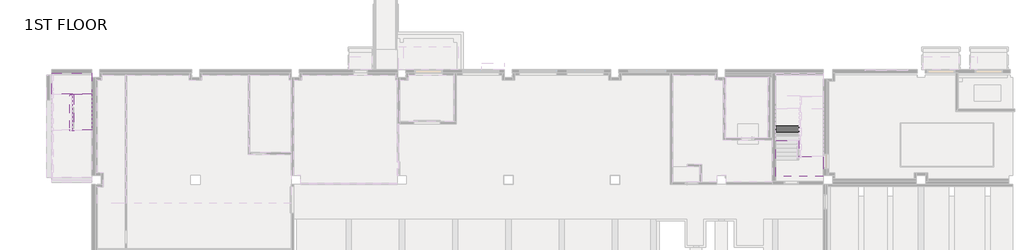
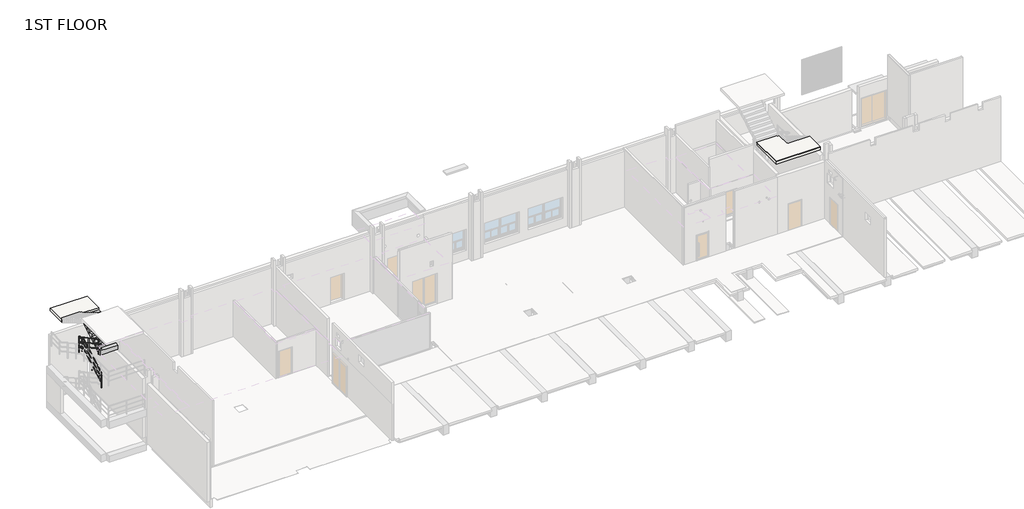
# One storey, part 13 of 15: 3 slabs, 2 stair flights, 1 railing.
"""IFC4 building model written with IfcOpenShell, lengths in millimetres."""

from ifc_helpers import new_model, si_unit, point, frame, frame_2d, origin, place, context, project, spatial, polyline, circle_curve, ellipse_curve, trimmed, segment, composite_curve, outline, extrude, faceted_brep, element, save
from ifc_brep_helpers import plane_surface, cylinder_surface, advanced_brep

model = new_model("IFC4")

# Units and contexts
model_context = context("Model", 3, world=origin())
ifc_project = project(units=[si_unit("LENGTHUNIT", "METRE", prefix="MILLI")], contexts=[model_context])

# Site, building, storey
site = spatial("IfcSite", under=ifc_project)
building = spatial("IfcBuilding", under=site)
storey = spatial("IfcBuildingStorey", under=building, Name="1ST FLOOR", Elevation=4800.0)

# Railing
placement = place(None, origin())
element("IfcRailing", 1, ObjectType="H_RL_AR_S10_Steel Handrail_H1200_STAIR", at=placement, inside=storey, context=model_context, shape_type="SolidModel", body=[
    advanced_brep(
    [(-1656.0, -4300.0, 8823.1475961), (-1694.0, -4300.0, 8823.1475961), (-1656.0, -1695.134128, 10251.0), (-1694.0, -1695.134128, 10251.0), (-1656.0, -1581.0, 10251.0), (-1694.0, -1619.0, 10251.0), (-1868.0, -1581.0, 10251.0), (-1868.0, -1619.0, 10251.0), (-1906.0, -1680.865872, 10402.2888889), (-1944.0, -1680.865872, 10402.2888889), (-1944.0, -4104.865872, 11731.0), (-1906.0, -4104.865872, 11731.0), (-1944.0, -4319.0, 11731.0), (-1906.0, -4281.0, 11731.0), (-1675.0, -4319.0, 11731.0), (-1675.0, -4281.0, 11731.0), (-1868.0, -1581.0, 10402.2888889), (-1868.0, -1619.0, 10402.2888889), (-1944.0, -1581.0, 10402.2888889), (-1906.0, -1619.0, 10402.2888889)],
    [
        (0, 1, ellipse_curve(frame((-1675.0, -4300.0, 8823.1475961), z_axis=(0.0, -1.0, 0.0), x_axis=(0.0, 0.0, -1.0)), 21.6672187, 19.0)),
        (1, 0, ellipse_curve(frame((-1675.0, -4300.0, 8823.1475961), z_axis=(0.0, -1.0, 0.0), x_axis=(0.0, 0.0, -1.0)), 21.6672187, 19.0)),
        (0, 2),
        (2, 3, ellipse_curve(frame((-1675.0, -1695.134128, 10251.0), z_axis=(0.0, -0.9687364795192938, -0.24809198545814556), x_axis=(0.0, 0.24809198545814448, -0.9687364795192941)), 19.613177, 19.0)),
        (3, 1),
        (3, 2, ellipse_curve(frame((-1675.0, -1695.134128, 10251.0), z_axis=(0.0, -0.9687364795192938, -0.24809198545814556), x_axis=(0.0, 0.24809198545814448, -0.9687364795192941)), 19.613177, 19.0)),
        (2, 4),
        (4, 5, ellipse_curve(frame((-1675.0, -1600.0, 10251.0), z_axis=(0.7071067811865467, -0.7071067811865485, 0.0), x_axis=(-0.7071067811865485, -0.7071067811865465, 0.0)), 26.8700577, 19.0)),
        (5, 3),
        (5, 4, ellipse_curve(frame((-1675.0, -1600.0, 10251.0), z_axis=(0.7071067811865467, -0.7071067811865485, 0.0), x_axis=(-0.7071067811865485, -0.7071067811865465, 0.0)), 26.8700577, 19.0)),
        (4, 6),
        (6, 7, ellipse_curve(frame((-1868.0, -1600.0, 10251.0), z_axis=(0.7071067811865475, 0.0, -0.7071067811865475), x_axis=(0.7071067811865477, 0.0, 0.7071067811865474)), 26.8700577, 19.0)),
        (7, 5),
        (7, 6, ellipse_curve(frame((-1868.0, -1600.0, 10251.0), z_axis=(0.7071067811865475, 0.0, -0.7071067811865475), x_axis=(0.7071067811865477, 0.0, 0.7071067811865474)), 26.8700577, 19.0)),
        (8, 9, ellipse_curve(frame((-1925.0, -1680.865872, 10402.2888889), z_axis=(0.0, -0.9687364795192939, 0.24809198545814537), x_axis=(0.0, -0.24809198545814468, -0.9687364795192942)), 19.613177, 19.0)),
        (9, 10),
        (10, 11, ellipse_curve(frame((-1925.0, -4104.865872, 11731.0), z_axis=(0.0, 0.9687364795192939, -0.24809198545814534), x_axis=(0.0, -0.24809198545814465, -0.9687364795192941)), 19.613177, 19.0)),
        (11, 8),
        (9, 8, ellipse_curve(frame((-1925.0, -1680.865872, 10402.2888889), z_axis=(0.0, -0.9687364795192939, 0.24809198545814537), x_axis=(0.0, -0.24809198545814468, -0.9687364795192942)), 19.613177, 19.0)),
        (11, 10, ellipse_curve(frame((-1925.0, -4104.865872, 11731.0), z_axis=(0.0, 0.9687364795192939, -0.24809198545814534), x_axis=(0.0, -0.24809198545814465, -0.9687364795192941)), 19.613177, 19.0)),
        (10, 12),
        (12, 13, ellipse_curve(frame((-1925.0, -4300.0, 11731.0), z_axis=(-0.7071067811864243, 0.7071067811866708, 0.0), x_axis=(0.7071067811866707, 0.7071067811864242, 0.0)), 26.8700577, 19.0)),
        (13, 11),
        (13, 12, ellipse_curve(frame((-1925.0, -4300.0, 11731.0), z_axis=(-0.7071067811864243, 0.7071067811866708, 0.0), x_axis=(0.7071067811866707, 0.7071067811864242, 0.0)), 26.8700577, 19.0)),
        (14, 15, circle_curve(frame((-1675.0, -4300.0, 11731.0), z_axis=(1.0, 0.0, 0.0), x_axis=(0.0, 1.0, 0.0)), 19.0)),
        (15, 14, circle_curve(frame((-1675.0, -4300.0, 11731.0), z_axis=(1.0, 0.0, 0.0), x_axis=(0.0, 1.0, 0.0)), 19.0)),
        (12, 14),
        (15, 13),
        (6, 16),
        (16, 17, ellipse_curve(frame((-1868.0, -1600.0, 10402.2888889), z_axis=(0.7071067811865475, 0.0, -0.7071067811865475), x_axis=(-0.7071067811865474, 0.0, -0.7071067811865476)), 26.8700577, 19.0)),
        (17, 7),
        (17, 16, ellipse_curve(frame((-1868.0, -1600.0, 10402.2888889), z_axis=(0.7071067811865475, 0.0, -0.7071067811865475), x_axis=(-0.7071067811865474, 0.0, -0.7071067811865476)), 26.8700577, 19.0)),
        (16, 18),
        (18, 19, ellipse_curve(frame((-1925.0, -1600.0, 10402.2888889), z_axis=(0.70710678118664, 0.707106781186455, 0.0), x_axis=(0.707106781186455, -0.70710678118664, 0.0)), 26.8700577, 19.0)),
        (19, 17),
        (19, 18, ellipse_curve(frame((-1925.0, -1600.0, 10402.2888889), z_axis=(0.70710678118664, 0.707106781186455, 0.0), x_axis=(0.707106781186455, -0.70710678118664, 0.0)), 26.8700577, 19.0)),
        (18, 9),
        (8, 19),
    ],
    [
        plane_surface(frame((-1675.0, -4300.0, 8844.8148148), z_axis=(0.0, -1.0, 0.0), x_axis=(0.0, 0.0, 1.0))),
        cylinder_surface(frame((-1675.0, -4290.8672412, 8828.1537009), z_axis=(0.0, -0.8769007335028707, -0.48067151317935164), x_axis=(-1.0, 0.0, 0.0)), 19.0),
        cylinder_surface(frame((-1675.0, -1700.0, 10251.0), z_axis=(0.0, -1.0, 0.0), x_axis=(-1.0, 0.0, 0.0)), 19.0),
        cylinder_surface(frame((-1675.0, -1600.0, 10251.0), z_axis=(1.0, 0.0, 0.0), x_axis=(0.0, -1.0, 0.0)), 19.0),
        cylinder_surface(frame((-1925.0, -1685.1327588, 10404.627775), z_axis=(0.0, 0.8769007335028708, -0.48067151317935125), x_axis=(1.0, 0.0, 0.0)), 19.0),
        cylinder_surface(frame((-1925.0, -4100.0, 11731.0), z_axis=(0.0, 1.0, 0.0), x_axis=(1.0, 0.0, 0.0)), 19.0),
        plane_surface(frame((-1675.0, -4300.0, 11750.0), z_axis=(1.0, 0.0, 0.0), x_axis=(0.0, 1.0, 0.0))),
        cylinder_surface(frame((-1925.0, -4300.0, 11731.0), z_axis=(-1.0, 0.0, 0.0), x_axis=(0.0, 1.0, 0.0)), 19.0),
        cylinder_surface(frame((-1868.0, -1600.0, 10270.0), z_axis=(0.0, 0.0, -1.0), x_axis=(0.0, -1.0, 0.0)), 19.0),
        cylinder_surface(frame((-1849.0, -1600.0, 10402.2888889), z_axis=(1.0, 0.0, 0.0), x_axis=(0.0, -1.0, 0.0)), 19.0),
        cylinder_surface(frame((-1925.0, -1600.0, 10402.2888889), z_axis=(0.0, 1.0, 0.0), x_axis=(1.0, 0.0, 0.0)), 19.0),
    ],
    [
        (0, [[1, 2]]),
        (1, [[-1, 3, 4, 5]]),
        (1, [[-2, -5, 6, -3]]),
        (2, [[-4, 7, 8, 9]]),
        (2, [[-6, -9, 10, -7]]),
        (3, [[-8, 11, 12, 13]]),
        (3, [[-10, -13, 14, -11]]),
        (4, [[15, 16, 17, 18]]),
        (4, [[19, -18, 20, -16]]),
        (5, [[-17, 21, 22, 23]]),
        (5, [[-20, -23, 24, -21]]),
        (6, [[25, 26]]),
        (7, [[-22, 27, -26, 28]]),
        (7, [[-24, -28, -25, -27]]),
        (8, [[-12, 29, 30, 31]]),
        (8, [[-14, -31, 32, -29]]),
        (9, [[-30, 33, 34, 35]]),
        (9, [[-32, -35, 36, -33]]),
        (10, [[-34, 37, -15, 38]]),
        (10, [[-36, -38, -19, -37]]),
    ],
),
    advanced_brep(
    [(-1675.0, -4319.0, 10931.0), (-1675.0, -4281.0, 10931.0), (-1944.0, -4319.0, 10931.0), (-1906.0, -4281.0, 10931.0)],
    [
        (0, 1, circle_curve(frame((-1675.0, -4300.0, 10931.0), z_axis=(1.0, 0.0, 0.0), x_axis=(0.0, 1.0, 0.0)), 19.0)),
        (1, 0, circle_curve(frame((-1675.0, -4300.0, 10931.0), z_axis=(1.0, 0.0, 0.0), x_axis=(0.0, 1.0, 0.0)), 19.0)),
        (2, 3, ellipse_curve(frame((-1925.0, -4300.0, 10931.0), z_axis=(-0.7071067811865471, 0.7071067811865479, 0.0), x_axis=(0.7071067811865479, 0.7071067811865471, 0.0)), 26.8700577, 19.0)),
        (3, 2, ellipse_curve(frame((-1925.0, -4300.0, 10931.0), z_axis=(-0.7071067811865471, 0.7071067811865479, 0.0), x_axis=(0.7071067811865479, 0.7071067811865471, 0.0)), 26.8700577, 19.0)),
        (0, 2),
        (3, 1),
    ],
    [
        plane_surface(frame((-1675.0, -4300.0, 10950.0), z_axis=(1.0, 0.0, 0.0), x_axis=(0.0, -1.0, 0.0))),
        plane_surface(frame((-1925.0, -4300.0, 10950.0), z_axis=(-0.7071067811865471, 0.7071067811865479, 0.0), x_axis=(0.7071067811865479, 0.7071067811865471, 0.0))),
        cylinder_surface(frame((-1675.0, -4300.0, 10931.0), z_axis=(1.0, 0.0, 0.0), x_axis=(0.0, 1.0, 0.0)), 19.0),
    ],
    [
        (0, [[1, 2]]),
        (1, [[3, 4]]),
        (2, [[-1, 5, -4, 6]]),
        (2, [[-2, -6, -3, -5]]),
    ],
),
    advanced_brep(
    [(-1944.0, -4319.0, 10931.0), (-1906.0, -4281.0, 10931.0), (-1944.0, -4104.865872, 10931.0), (-1906.0, -4104.865872, 10931.0), (-1944.0, -1592.4716448, 9553.8357569), (-1906.0, -1625.7938727, 9572.1012744)],
    [
        (0, 1, ellipse_curve(frame((-1925.0, -4300.0, 10931.0), z_axis=(0.7071067811865471, -0.7071067811865479, 0.0), x_axis=(-0.7071067811865478, -0.7071067811865472, 0.0)), 26.8700577, 19.0)),
        (1, 0, ellipse_curve(frame((-1925.0, -4300.0, 10931.0), z_axis=(0.7071067811865471, -0.7071067811865479, 0.0), x_axis=(-0.7071067811865478, -0.7071067811865472, 0.0)), 26.8700577, 19.0)),
        (0, 2),
        (2, 3, ellipse_curve(frame((-1925.0, -4104.865872, 10931.0), z_axis=(0.0, -0.9687364795192939, 0.24809198545814531), x_axis=(0.0, -0.24809198545814604, -0.9687364795192938)), 19.613177, 19.0)),
        (3, 1),
        (3, 2, ellipse_curve(frame((-1925.0, -4104.865872, 10931.0), z_axis=(0.0, -0.9687364795192939, 0.24809198545814531), x_axis=(0.0, -0.24809198545814604, -0.9687364795192938)), 19.613177, 19.0)),
        (4, 5, ellipse_curve(frame((-1925.0, -1609.1327588, 9562.9685157), z_axis=(0.7071067811865346, 0.6200624550873559, -0.33988608649231156), x_axis=(0.7071067811865606, -0.6200624550873189, 0.33988608649232477)), 26.8700577, 19.0)),
        (5, 4, ellipse_curve(frame((-1925.0, -1609.1327588, 9562.9685157), z_axis=(0.7071067811865346, 0.6200624550873559, -0.33988608649231156), x_axis=(0.7071067811865606, -0.6200624550873189, 0.33988608649232477)), 26.8700577, 19.0)),
        (2, 4),
        (5, 3),
    ],
    [
        plane_surface(frame((-1925.0, -4300.0, 10950.0), z_axis=(0.7071067811865471, -0.7071067811865479, 0.0), x_axis=(0.7071067811865479, 0.7071067811865471, 0.0))),
        cylinder_surface(frame((-1925.0, -4300.0, 10931.0), z_axis=(0.0, -1.0, 0.0), x_axis=(1.0, 0.0, 0.0)), 19.0),
        plane_surface(frame((-1925.0, -1600.0, 9579.6296296), z_axis=(0.7071067811865346, 0.6200624550873559, -0.33988608649231156), x_axis=(0.7071067811865605, -0.6200624550873332, 0.33988608649229907))),
        cylinder_surface(frame((-1925.0, -4109.1327588, 10933.3388861), z_axis=(0.0, -0.8769007335028708, 0.4806715131793512), x_axis=(1.0, 0.0, 0.0)), 19.0),
    ],
    [
        (0, [[1, 2]]),
        (1, [[-1, 3, 4, 5]]),
        (1, [[-2, -5, 6, -3]]),
        (2, [[7, 8]]),
        (3, [[-4, 9, -8, 10]]),
        (3, [[-6, -10, -7, -9]]),
    ],
),
    advanced_brep(
    [(-1950.7938727, -1581.0, 9451.0), (-1917.4716448, -1619.0, 9451.0), (-1656.0, -1581.0, 9451.0), (-1694.0, -1619.0, 9451.0)],
    [
        (0, 1, ellipse_curve(frame((-1934.1327587, -1600.0, 9451.0), z_axis=(-0.7071067811865346, -0.6200624550873559, 0.33988608649231156), x_axis=(-0.7071067811865603, 0.6200624550873332, -0.33988608649229907)), 26.8700577, 19.0)),
        (1, 0, ellipse_curve(frame((-1934.1327587, -1600.0, 9451.0), z_axis=(-0.7071067811865346, -0.6200624550873559, 0.33988608649231156), x_axis=(-0.7071067811865603, 0.6200624550873332, -0.33988608649229907)), 26.8700577, 19.0)),
        (2, 3, ellipse_curve(frame((-1675.0, -1600.0, 9451.0), z_axis=(0.7071067811865619, -0.7071067811865331, 0.0), x_axis=(-0.7071067811865331, -0.7071067811865619, 0.0)), 26.8700577, 19.0)),
        (3, 2, ellipse_curve(frame((-1675.0, -1600.0, 9451.0), z_axis=(0.7071067811865619, -0.7071067811865331, 0.0), x_axis=(-0.7071067811865331, -0.7071067811865619, 0.0)), 26.8700577, 19.0)),
        (0, 2),
        (3, 1),
    ],
    [
        plane_surface(frame((-1925.0, -1600.0, 9470.0), z_axis=(-0.7071067811865346, -0.6200624550873559, 0.33988608649231156), x_axis=(0.7071067811865605, -0.6200624550873332, 0.33988608649229907))),
        plane_surface(frame((-1675.0, -1600.0, 9470.0), z_axis=(0.7071067811865619, -0.7071067811865331, 0.0), x_axis=(0.7071067811865331, 0.7071067811865619, 0.0))),
        cylinder_surface(frame((-1925.0, -1600.0, 9451.0), z_axis=(-1.0, 0.0, 0.0), x_axis=(0.0, -1.0, 0.0)), 19.0),
    ],
    [
        (0, [[1, 2]]),
        (1, [[3, 4]]),
        (2, [[-1, 5, -4, 6]]),
        (2, [[-2, -6, -3, -5]]),
    ],
),
    advanced_brep(
    [(-1656.0, -1581.0, 9451.0), (-1694.0, -1619.0, 9451.0), (-1656.0, -1695.134128, 9451.0), (-1694.0, -1695.134128, 9451.0), (-1656.0, -4300.0, 8023.1475961), (-1694.0, -4300.0, 8023.1475961)],
    [
        (0, 1, ellipse_curve(frame((-1675.0, -1600.0, 9451.0), z_axis=(-0.7071067811865619, 0.7071067811865331, 0.0), x_axis=(0.707106781186533, 0.7071067811865619, 0.0)), 26.8700577, 19.0)),
        (1, 0, ellipse_curve(frame((-1675.0, -1600.0, 9451.0), z_axis=(-0.7071067811865619, 0.7071067811865331, 0.0), x_axis=(0.707106781186533, 0.7071067811865619, 0.0)), 26.8700577, 19.0)),
        (0, 2),
        (2, 3, ellipse_curve(frame((-1675.0, -1695.134128, 9451.0), z_axis=(0.0, 0.9687364795192939, 0.24809198545814562), x_axis=(0.0, 0.24809198545814576, -0.9687364795192939)), 19.613177, 19.0)),
        (3, 1),
        (3, 2, ellipse_curve(frame((-1675.0, -1695.134128, 9451.0), z_axis=(0.0, 0.9687364795192939, 0.24809198545814562), x_axis=(0.0, 0.24809198545814576, -0.9687364795192939)), 19.613177, 19.0)),
        (4, 5, ellipse_curve(frame((-1675.0, -4300.0, 8023.1475961), z_axis=(0.0, -1.0, 0.0), x_axis=(0.0, 0.0, 0.9999999999999999)), 21.6672187, 19.0)),
        (5, 4, ellipse_curve(frame((-1675.0, -4300.0, 8023.1475961), z_axis=(0.0, -1.0, 0.0), x_axis=(0.0, 0.0, 0.9999999999999999)), 21.6672187, 19.0)),
        (2, 4),
        (5, 3),
    ],
    [
        plane_surface(frame((-1675.0, -1600.0, 9470.0), z_axis=(-0.7071067811865619, 0.7071067811865331, 0.0), x_axis=(0.7071067811865331, 0.7071067811865619, 0.0))),
        cylinder_surface(frame((-1675.0, -1600.0, 9451.0), z_axis=(0.0, 1.0, 0.0), x_axis=(-1.0, 0.0, 0.0)), 19.0),
        plane_surface(frame((-1675.0, -4300.0, 8044.8148148), z_axis=(0.0, -1.0, 0.0), x_axis=(0.0, 0.0, -1.0))),
        cylinder_surface(frame((-1675.0, -1690.8672412, 9453.3388861), z_axis=(0.0, 0.8769007335028706, 0.4806715131793517), x_axis=(-1.0, 0.0, 0.0)), 19.0),
    ],
    [
        (0, [[1, 2]]),
        (1, [[-1, 3, 4, 5]]),
        (1, [[-2, -5, 6, -3]]),
        (2, [[7, 8]]),
        (3, [[-4, 9, -8, 10]]),
        (3, [[-6, -10, -7, -9]]),
    ],
),
    advanced_brep(
    [(-1675.0, -4319.0, 11331.0), (-1675.0, -4281.0, 11331.0), (-1944.0, -4319.0, 11331.0), (-1906.0, -4281.0, 11331.0)],
    [
        (0, 1, circle_curve(frame((-1675.0, -4300.0, 11331.0), z_axis=(1.0, 0.0, 0.0), x_axis=(0.0, 1.0, 0.0)), 19.0)),
        (1, 0, circle_curve(frame((-1675.0, -4300.0, 11331.0), z_axis=(1.0, 0.0, 0.0), x_axis=(0.0, 1.0, 0.0)), 19.0)),
        (2, 3, ellipse_curve(frame((-1925.0, -4300.0, 11331.0), z_axis=(-0.7071067811865471, 0.7071067811865479, 0.0), x_axis=(0.7071067811865479, 0.7071067811865471, 0.0)), 26.8700577, 19.0)),
        (3, 2, ellipse_curve(frame((-1925.0, -4300.0, 11331.0), z_axis=(-0.7071067811865471, 0.7071067811865479, 0.0), x_axis=(0.7071067811865479, 0.7071067811865471, 0.0)), 26.8700577, 19.0)),
        (0, 2),
        (3, 1),
    ],
    [
        plane_surface(frame((-1675.0, -4300.0, 11350.0), z_axis=(1.0, 0.0, 0.0), x_axis=(0.0, -1.0, 0.0))),
        plane_surface(frame((-1925.0, -4300.0, 11350.0), z_axis=(-0.7071067811865471, 0.7071067811865479, 0.0), x_axis=(0.7071067811865479, 0.7071067811865471, 0.0))),
        cylinder_surface(frame((-1675.0, -4300.0, 11331.0), z_axis=(1.0, 0.0, 0.0), x_axis=(0.0, 1.0, 0.0)), 19.0),
    ],
    [
        (0, [[1, 2]]),
        (1, [[3, 4]]),
        (2, [[-1, 5, -4, 6]]),
        (2, [[-2, -6, -3, -5]]),
    ],
),
    advanced_brep(
    [(-1944.0, -4319.0, 11331.0), (-1906.0, -4281.0, 11331.0), (-1944.0, -4104.865872, 11331.0), (-1906.0, -4104.865872, 11331.0), (-1944.0, -1592.4716448, 9953.8357569), (-1906.0, -1625.7938727, 9972.1012744)],
    [
        (0, 1, ellipse_curve(frame((-1925.0, -4300.0, 11331.0), z_axis=(0.7071067811865471, -0.7071067811865479, 0.0), x_axis=(-0.7071067811865478, -0.7071067811865472, 0.0)), 26.8700577, 19.0)),
        (1, 0, ellipse_curve(frame((-1925.0, -4300.0, 11331.0), z_axis=(0.7071067811865471, -0.7071067811865479, 0.0), x_axis=(-0.7071067811865478, -0.7071067811865472, 0.0)), 26.8700577, 19.0)),
        (0, 2),
        (2, 3, ellipse_curve(frame((-1925.0, -4104.865872, 11331.0), z_axis=(0.0, -0.9687364795192939, 0.24809198545814531), x_axis=(0.0, -0.24809198545814604, -0.9687364795192938)), 19.613177, 19.0)),
        (3, 1),
        (3, 2, ellipse_curve(frame((-1925.0, -4104.865872, 11331.0), z_axis=(0.0, -0.9687364795192939, 0.24809198545814531), x_axis=(0.0, -0.24809198545814604, -0.9687364795192938)), 19.613177, 19.0)),
        (4, 5, ellipse_curve(frame((-1925.0, -1609.1327588, 9962.9685157), z_axis=(0.7071067811865346, 0.6200624550873559, -0.33988608649231156), x_axis=(0.7071067811865606, -0.6200624550873189, 0.33988608649232477)), 26.8700577, 19.0)),
        (5, 4, ellipse_curve(frame((-1925.0, -1609.1327588, 9962.9685157), z_axis=(0.7071067811865346, 0.6200624550873559, -0.33988608649231156), x_axis=(0.7071067811865606, -0.6200624550873189, 0.33988608649232477)), 26.8700577, 19.0)),
        (2, 4),
        (5, 3),
    ],
    [
        plane_surface(frame((-1925.0, -4300.0, 11350.0), z_axis=(0.7071067811865471, -0.7071067811865479, 0.0), x_axis=(0.7071067811865479, 0.7071067811865471, 0.0))),
        cylinder_surface(frame((-1925.0, -4300.0, 11331.0), z_axis=(0.0, -1.0, 0.0), x_axis=(1.0, 0.0, 0.0)), 19.0),
        plane_surface(frame((-1925.0, -1600.0, 9979.6296296), z_axis=(0.7071067811865346, 0.6200624550873559, -0.33988608649231156), x_axis=(0.7071067811865605, -0.6200624550873332, 0.33988608649229907))),
        cylinder_surface(frame((-1925.0, -4109.1327588, 11333.3388861), z_axis=(0.0, -0.8769007335028708, 0.4806715131793512), x_axis=(1.0, 0.0, 0.0)), 19.0),
    ],
    [
        (0, [[1, 2]]),
        (1, [[-1, 3, 4, 5]]),
        (1, [[-2, -5, 6, -3]]),
        (2, [[7, 8]]),
        (3, [[-4, 9, -8, 10]]),
        (3, [[-6, -10, -7, -9]]),
    ],
),
    advanced_brep(
    [(-1950.7938727, -1581.0, 9851.0), (-1917.4716448, -1619.0, 9851.0), (-1656.0, -1581.0, 9851.0), (-1694.0, -1619.0, 9851.0)],
    [
        (0, 1, ellipse_curve(frame((-1934.1327587, -1600.0, 9851.0), z_axis=(-0.7071067811865346, -0.6200624550873559, 0.33988608649231156), x_axis=(-0.7071067811865603, 0.6200624550873332, -0.33988608649229907)), 26.8700577, 19.0)),
        (1, 0, ellipse_curve(frame((-1934.1327587, -1600.0, 9851.0), z_axis=(-0.7071067811865346, -0.6200624550873559, 0.33988608649231156), x_axis=(-0.7071067811865603, 0.6200624550873332, -0.33988608649229907)), 26.8700577, 19.0)),
        (2, 3, ellipse_curve(frame((-1675.0, -1600.0, 9851.0), z_axis=(0.7071067811865619, -0.7071067811865331, 0.0), x_axis=(-0.7071067811865331, -0.7071067811865619, 0.0)), 26.8700577, 19.0)),
        (3, 2, ellipse_curve(frame((-1675.0, -1600.0, 9851.0), z_axis=(0.7071067811865619, -0.7071067811865331, 0.0), x_axis=(-0.7071067811865331, -0.7071067811865619, 0.0)), 26.8700577, 19.0)),
        (0, 2),
        (3, 1),
    ],
    [
        plane_surface(frame((-1925.0, -1600.0, 9870.0), z_axis=(-0.7071067811865346, -0.6200624550873559, 0.33988608649231156), x_axis=(0.7071067811865605, -0.6200624550873332, 0.33988608649229907))),
        plane_surface(frame((-1675.0, -1600.0, 9870.0), z_axis=(0.7071067811865619, -0.7071067811865331, 0.0), x_axis=(0.7071067811865331, 0.7071067811865619, 0.0))),
        cylinder_surface(frame((-1925.0, -1600.0, 9851.0), z_axis=(-1.0, 0.0, 0.0), x_axis=(0.0, -1.0, 0.0)), 19.0),
    ],
    [
        (0, [[1, 2]]),
        (1, [[3, 4]]),
        (2, [[-1, 5, -4, 6]]),
        (2, [[-2, -6, -3, -5]]),
    ],
),
    advanced_brep(
    [(-1656.0, -1581.0, 9851.0), (-1694.0, -1619.0, 9851.0), (-1656.0, -1695.134128, 9851.0), (-1694.0, -1695.134128, 9851.0), (-1656.0, -4300.0, 8423.1475961), (-1694.0, -4300.0, 8423.1475961)],
    [
        (0, 1, ellipse_curve(frame((-1675.0, -1600.0, 9851.0), z_axis=(-0.7071067811865619, 0.7071067811865331, 0.0), x_axis=(0.707106781186533, 0.7071067811865619, 0.0)), 26.8700577, 19.0)),
        (1, 0, ellipse_curve(frame((-1675.0, -1600.0, 9851.0), z_axis=(-0.7071067811865619, 0.7071067811865331, 0.0), x_axis=(0.707106781186533, 0.7071067811865619, 0.0)), 26.8700577, 19.0)),
        (0, 2),
        (2, 3, ellipse_curve(frame((-1675.0, -1695.134128, 9851.0), z_axis=(0.0, 0.9687364795192939, 0.24809198545814562), x_axis=(0.0, 0.24809198545814576, -0.9687364795192939)), 19.613177, 19.0)),
        (3, 1),
        (3, 2, ellipse_curve(frame((-1675.0, -1695.134128, 9851.0), z_axis=(0.0, 0.9687364795192939, 0.24809198545814562), x_axis=(0.0, 0.24809198545814576, -0.9687364795192939)), 19.613177, 19.0)),
        (4, 5, ellipse_curve(frame((-1675.0, -4300.0, 8423.1475961), z_axis=(0.0, -1.0, 0.0), x_axis=(0.0, 0.0, 0.9999999999999999)), 21.6672187, 19.0)),
        (5, 4, ellipse_curve(frame((-1675.0, -4300.0, 8423.1475961), z_axis=(0.0, -1.0, 0.0), x_axis=(0.0, 0.0, 0.9999999999999999)), 21.6672187, 19.0)),
        (2, 4),
        (5, 3),
    ],
    [
        plane_surface(frame((-1675.0, -1600.0, 9870.0), z_axis=(-0.7071067811865619, 0.7071067811865331, 0.0), x_axis=(0.7071067811865331, 0.7071067811865619, 0.0))),
        cylinder_surface(frame((-1675.0, -1600.0, 9851.0), z_axis=(0.0, 1.0, 0.0), x_axis=(-1.0, 0.0, 0.0)), 19.0),
        plane_surface(frame((-1675.0, -4300.0, 8444.8148148), z_axis=(0.0, -1.0, 0.0), x_axis=(0.0, 0.0, -1.0))),
        cylinder_surface(frame((-1675.0, -1690.8672412, 9853.3388861), z_axis=(0.0, 0.8769007335028706, 0.4806715131793517), x_axis=(-1.0, 0.0, 0.0)), 19.0),
    ],
    [
        (0, [[1, 2]]),
        (1, [[-1, 3, 4, 5]]),
        (1, [[-2, -5, 6, -3]]),
        (2, [[7, 8]]),
        (3, [[-4, 9, -8, 10]]),
        (3, [[-6, -10, -7, -9]]),
    ],
),
    advanced_brep(
    [(-1696.2, -4300.0, 8801.4803773), (-1696.2, -4300.0, 7590.0), (-1653.8, -4300.0, 7590.0), (-1653.8, -4300.0, 8801.4803773)],
    [
        (0, 1),
        (1, 2, circle_curve(frame((-1675.0, -4300.0, 7590.0), z_axis=(0.0, 0.0, 1.0), x_axis=(1.0, 0.0, 0.0)), 21.2)),
        (2, 3),
        (3, 0, ellipse_curve(frame((-1675.0, -4300.0, 8801.4803773), z_axis=(0.0, 0.4806715131793478, -0.8769007335028728), x_axis=(0.0, 0.8769007335028729, 0.4806715131793474)), 24.1760546, 21.2)),
        (0, 3, ellipse_curve(frame((-1675.0, -4300.0, 8801.4803773), z_axis=(0.0, 0.4806715131793478, -0.8769007335028728), x_axis=(0.0, 0.8769007335028729, 0.4806715131793474)), 24.1760546, 21.2)),
        (2, 1, circle_curve(frame((-1675.0, -4300.0, 7590.0), z_axis=(0.0, 0.0, 1.0), x_axis=(1.0, 0.0, 0.0)), 21.2)),
    ],
    [
        cylinder_surface(frame((-1675.0, -4300.0, 7490.0), z_axis=(0.0, 0.0, 1.0), x_axis=(1.0, 0.0, 0.0)), 21.2),
        plane_surface(frame((-1650.0, -4325.0, 8787.7766736), z_axis=(0.0, -0.4806715131793478, 0.8769007335028728), x_axis=(-1.0, 0.0, 0.0))),
        plane_surface(frame((-1650.0, -4275.0, 7590.0), z_axis=(0.0, 0.0, -1.0), x_axis=(-1.0, 0.0, 0.0))),
    ],
    [
        (0, [[1, 2, 3, 4]]),
        (0, [[-1, 5, -3, 6]]),
        (1, [[-4, -5]]),
        (2, [[-2, -6]]),
    ],
),
    advanced_brep(
    [(-1696.2, -2950.0, 9541.4803773), (-1696.2, -2950.0, 8247.7777778), (-1653.8, -2950.0, 8247.7777778), (-1653.8, -2950.0, 9541.4803773)],
    [
        (0, 1),
        (1, 2, circle_curve(frame((-1675.0, -2950.0, 8247.7777778), z_axis=(0.0, 0.0, 1.0), x_axis=(1.0, 0.0, 0.0)), 21.2)),
        (2, 3),
        (3, 0, ellipse_curve(frame((-1675.0, -2950.0, 9541.4803773), z_axis=(0.0, 0.4806715131793496, -0.8769007335028717), x_axis=(0.0, 0.8769007335028718, 0.4806715131793496)), 24.1760546, 21.2)),
        (0, 3, ellipse_curve(frame((-1675.0, -2950.0, 9541.4803773), z_axis=(0.0, 0.4806715131793496, -0.8769007335028717), x_axis=(0.0, 0.8769007335028718, 0.4806715131793496)), 24.1760546, 21.2)),
        (2, 1, circle_curve(frame((-1675.0, -2950.0, 8247.7777778), z_axis=(0.0, 0.0, 1.0), x_axis=(1.0, 0.0, 0.0)), 21.2)),
    ],
    [
        cylinder_surface(frame((-1675.0, -2950.0, 8147.7777778), z_axis=(0.0, 0.0, 1.0), x_axis=(1.0, 0.0, 0.0)), 21.2),
        plane_surface(frame((-1650.0, -2975.0, 9527.7766736), z_axis=(0.0, -0.4806715131793496, 0.8769007335028717), x_axis=(-1.0, 0.0, 0.0))),
        plane_surface(frame((-1650.0, -2925.0, 8247.7777778), z_axis=(0.0, 0.0, -1.0), x_axis=(-1.0, 0.0, 0.0))),
    ],
    [
        (0, [[1, 2, 3, 4]]),
        (0, [[-1, 5, -3, 6]]),
        (1, [[-4, -5]]),
        (2, [[-2, -6]]),
    ],
),
    extrude(outline(composite_curve([segment(trimmed(circle_curve(frame_2d((-1675.0, -1600.0)), 21.2), [point((-1653.8, -1600.0))], [point((-1696.2, -1600.0))], False, "CARTESIAN"), True, "CONTINUOUS"), segment(trimmed(circle_curve(frame_2d((-1675.0, -1600.0)), 21.2), [point((-1696.2, -1600.0))], [point((-1653.8, -1600.0))], False, "CARTESIAN"), True, "CONTINUOUS")], self_intersect=False)), frame((0.0, 0.0, 9070.0), z_axis=(0.0, 0.0, 1.0), x_axis=(1.0, 0.0, 0.0)), (0.0, 0.0, 1.0), 1162.0),
    extrude(outline(composite_curve([segment(trimmed(circle_curve(frame_2d((-1925.0, -1600.0)), 21.2), [point((-1946.2, -1600.0))], [point((-1903.8, -1600.0))], False, "CARTESIAN"), True, "CONTINUOUS"), segment(trimmed(circle_curve(frame_2d((-1925.0, -1600.0)), 21.2), [point((-1903.8, -1600.0))], [point((-1946.2, -1600.0))], False, "CARTESIAN"), True, "CONTINUOUS")], self_intersect=False)), frame((0.0, 0.0, 9070.0), z_axis=(0.0, 0.0, 1.0), x_axis=(1.0, 0.0, 0.0)), (0.0, 0.0, 1.0), 1313.2888889),
    advanced_brep(
    [(-1903.8, -2950.0, 11076.2951922), (-1903.8, -2950.0, 9892.2222222), (-1946.2, -2950.0, 9892.2222222), (-1946.2, -2950.0, 11076.2951922)],
    [
        (0, 1),
        (1, 2, circle_curve(frame((-1925.0, -2950.0, 9892.2222222), z_axis=(0.0, 0.0, 1.0), x_axis=(-1.0, 0.0, 0.0)), 21.2)),
        (2, 3),
        (3, 0, ellipse_curve(frame((-1925.0, -2950.0, 11076.2951922), z_axis=(0.0, -0.4806715131793478, -0.8769007335028728), x_axis=(0.0, -0.8769007335028729, 0.4806715131793474)), 24.1760546, 21.2)),
        (0, 3, ellipse_curve(frame((-1925.0, -2950.0, 11076.2951922), z_axis=(0.0, -0.4806715131793478, -0.8769007335028728), x_axis=(0.0, -0.8769007335028729, 0.4806715131793474)), 24.1760546, 21.2)),
        (2, 1, circle_curve(frame((-1925.0, -2950.0, 9892.2222222), z_axis=(0.0, 0.0, 1.0), x_axis=(-1.0, 0.0, 0.0)), 21.2)),
    ],
    [
        cylinder_surface(frame((-1925.0, -2950.0, 9792.2222222), z_axis=(0.0, 0.0, 1.0), x_axis=(-1.0, 0.0, 0.0)), 21.2),
        plane_surface(frame((-1950.0, -2925.0, 11062.5914885), z_axis=(0.0, 0.4806715131793478, 0.8769007335028728), x_axis=(1.0, 0.0, 0.0))),
        plane_surface(frame((-1950.0, -2975.0, 9892.2222222), z_axis=(0.0, 0.0, -1.0), x_axis=(1.0, 0.0, 0.0))),
    ],
    [
        (0, [[1, 2, 3, 4]]),
        (0, [[-1, 5, -3, 6]]),
        (1, [[-4, -5]]),
        (2, [[-2, -6]]),
    ],
),
    extrude(outline(composite_curve([segment(trimmed(circle_curve(frame_2d((-1925.0, -4300.0)), 21.2), [point((-1946.2, -4300.0))], [point((-1903.8, -4300.0))], False, "CARTESIAN"), True, "CONTINUOUS"), segment(trimmed(circle_curve(frame_2d((-1925.0, -4300.0)), 21.2), [point((-1903.8, -4300.0))], [point((-1946.2, -4300.0))], False, "CARTESIAN"), True, "CONTINUOUS")], self_intersect=False)), frame((0.0, 0.0, 10550.0), z_axis=(0.0, 0.0, 1.0), x_axis=(1.0, 0.0, 0.0)), (0.0, 0.0, 1.0), 1162.0),
])

# Slabs
element("IfcSlab", 2, ObjectType="H_FL_AR_S17_RC Slab_T200_SS1", at=placement, inside=storey, context=model_context, shape_type="Brep", body=[
    faceted_brep([(-1750.0, -1550.0, 12300.0), (-300.0, -1550.0, 12300.0), (-300.0, -1195.9301717, 12300.0), (-300.0, 50.0, 12300.0), (-3300.0, 50.0, 12300.0), (-3300.0, -1550.0, 12300.0), (-1850.0, -1550.0, 12300.0), (-1750.0, -1550.0, 12100.0), (-1750.0, -1550.0, 11893.4592668), (-300.0, -1550.0, 11893.4592668), (-300.0, -1195.9301717, 12100.0), (-300.0, 50.0, 12100.0), (-3300.0, 50.0, 12100.0), (-3300.0, -1550.0, 12100.0), (-1850.0, -1550.0, 12100.0), (-1750.0, -1195.9301717, 12100.0)], [[[0, 1, 2, 3, 4, 5, 6]], [[1, 0, 7, 8, 9]], [[1, 9, 10, 11, 3, 2]], [[4, 3, 11, 12]], [[5, 4, 12, 13]], [[6, 5, 13, 14]], [[0, 6, 14, 7]], [[10, 15, 7, 14, 13, 12, 11]], [[15, 10, 9, 8]], [[7, 15, 8]]]),
])
element("IfcSlab", 3, ObjectType="H_FL_AR_S17_RC Slab_T200_SS1", at=placement, inside=storey, context=model_context, shape_type="Brep", body=[
    faceted_brep([(54650.0, -6230.0, 10570.0), (52915.0, -6230.0, 10570.0), (52810.0, -6230.0, 10570.0), (52810.0, -5020.0, 10570.0), (51075.0149406, -5020.0, 10570.0), (51075.0149406, -7750.0, 10570.0), (54650.0, -7750.0, 10570.0), (54650.0, -6585.2317377, 10570.0), (54650.0, -6230.0, 10157.6010235), (54650.0, -7750.0, 10370.0), (54650.0, -6585.2317377, 10370.0), (52810.0, -6230.0, 10370.0), (52810.0, -5020.0, 10370.0), (51075.0149406, -5020.0, 10370.0), (51075.0149406, -7750.0, 10370.0), (52915.0, -6585.2317377, 10370.0), (52915.0, -6230.0, 10370.0), (52915.0, -6230.0, 10157.6010235)], [[[0, 1, 2, 3, 4, 5, 6, 7]], [[8, 0, 7, 6, 9, 10]], [[3, 2, 11, 12]], [[4, 3, 12, 13]], [[5, 4, 13, 14]], [[6, 5, 14, 9]], [[15, 10, 9, 14, 13, 12, 11, 16]], [[1, 0, 8, 17, 16]], [[2, 1, 16, 11]], [[10, 15, 17, 8]], [[15, 16, 17]]]),
])
element("IfcSlab", 4, ObjectType="Deco Tile", at=placement, inside=storey, context=model_context, shape_type="SweptSolid", body=[
    extrude(outline(polyline([(52915.0, -6230.0), (54650.0, -6230.0), (54650.0, -7750.0), (51075.0, -7750.0), (51075.0, -5020.0), (52810.0, -5020.0), (52810.0, -6200.0), (52914.0012627, -6200.0), (52915.0, -6200.0), (52915.0, -6230.0)])), frame((0.0, 0.0, 10570.0), z_axis=(0.0, 0.0, 1.0), x_axis=(1.0, 0.0, 0.0)), (0.0, 0.0, 1.0), 30.0),
])

# Stair flights
element("IfcStairFlight", 5, ObjectType="Concrete", at=placement, inside=storey, context=model_context, shape_type="Brep", body=[
    faceted_brep([(-1750.0, -3950.0, 10725.0), (-1750.0, -4250.0, 10725.0), (-300.0, -4250.0, 10725.0), (-300.0, -3950.0, 10725.0), (-1750.0, -3950.0, 10493.4592668), (-1750.0, -4195.9301717, 10350.0), (-1750.0, -4250.0, 10350.0), (-300.0, -4250.0, 10350.0), (-300.0, -4195.9301717, 10350.0), (-300.0, -3950.0, 10493.4592668), (-1750.0, -3650.0, 10900.0), (-1750.0, -3950.0, 10900.0), (-300.0, -3950.0, 10900.0), (-300.0, -3650.0, 10900.0), (-1750.0, -3650.0, 10668.4592668), (-300.0, -3650.0, 10668.4592668), (-1750.0, -3350.0, 11075.0), (-1750.0, -3650.0, 11075.0), (-300.0, -3650.0, 11075.0), (-300.0, -3350.0, 11075.0), (-1750.0, -3350.0, 10843.4592668), (-300.0, -3350.0, 10843.4592668), (-1750.0, -3050.0, 11250.0), (-1750.0, -3350.0, 11250.0), (-300.0, -3350.0, 11250.0), (-300.0, -3050.0, 11250.0), (-1750.0, -3050.0, 11018.4592668), (-300.0, -3050.0, 11018.4592668), (-1750.0, -2750.0, 11425.0), (-1750.0, -3050.0, 11425.0), (-300.0, -3050.0, 11425.0), (-300.0, -2750.0, 11425.0), (-1750.0, -2750.0, 11193.4592668), (-300.0, -2750.0, 11193.4592668), (-1750.0, -2450.0, 11600.0), (-1750.0, -2750.0, 11600.0), (-300.0, -2750.0, 11600.0), (-300.0, -2450.0, 11600.0), (-1750.0, -2450.0, 11368.4592668), (-300.0, -2450.0, 11368.4592668), (-1750.0, -2150.0, 11775.0), (-1750.0, -2450.0, 11775.0), (-300.0, -2450.0, 11775.0), (-300.0, -2150.0, 11775.0), (-1750.0, -2150.0, 11543.4592668), (-300.0, -2150.0, 11543.4592668), (-1750.0, -1850.0, 11950.0), (-1750.0, -2150.0, 11950.0), (-300.0, -2150.0, 11950.0), (-300.0, -1850.0, 11950.0), (-1750.0, -1850.0, 11718.4592668), (-300.0, -1850.0, 11718.4592668), (-1750.0, -1550.0, 11893.4592668), (-300.0, -1550.0, 11893.4592668), (-1750.0, -1550.0, 12125.0), (-1750.0, -1850.0, 12125.0), (-300.0, -1850.0, 12125.0), (-300.0, -1550.0, 12125.0), (-1750.0, -1550.0, 12100.0)], [[[0, 1, 2, 3]], [[1, 0, 4, 5, 6]], [[2, 1, 6, 7]], [[3, 2, 7, 8, 9]], [[10, 11, 12, 13]], [[11, 10, 14, 4, 0]], [[0, 3, 12, 11]], [[13, 12, 3, 9, 15]], [[16, 17, 18, 19]], [[17, 16, 20, 14, 10]], [[10, 13, 18, 17]], [[19, 18, 13, 15, 21]], [[22, 23, 24, 25]], [[23, 22, 26, 20, 16]], [[16, 19, 24, 23]], [[25, 24, 19, 21, 27]], [[28, 29, 30, 31]], [[29, 28, 32, 26, 22]], [[22, 25, 30, 29]], [[31, 30, 25, 27, 33]], [[34, 35, 36, 37]], [[35, 34, 38, 32, 28]], [[28, 31, 36, 35]], [[37, 36, 31, 33, 39]], [[40, 41, 42, 43]], [[41, 40, 44, 38, 34]], [[34, 37, 42, 41]], [[43, 42, 37, 39, 45]], [[46, 47, 48, 49]], [[47, 46, 50, 44, 40]], [[40, 43, 48, 47]], [[49, 48, 43, 45, 51]], [[7, 6, 5, 8]], [[8, 5, 4, 14, 20, 26, 32, 38, 44, 50, 52, 53, 51, 45, 39, 33, 27, 21, 15, 9]], [[54, 55, 56, 57]], [[55, 54, 58, 52, 50, 46]], [[46, 49, 56, 55]], [[57, 56, 49, 51, 53]], [[54, 57, 53, 52, 58]]]),
])
element("IfcStairFlight", 6, ObjectType="Concrete", at=placement, inside=storey, context=model_context, shape_type="Brep", body=[
    faceted_brep([(51075.0, -6170.0, 4970.5882353), (51075.0, -6470.0, 4970.5882353), (52810.0, -6470.0, 4970.5882353), (52810.0, -6170.0, 4970.5882353), (51075.0, -6170.0, 4800.0), (51075.0, -6470.0, 4800.0), (52810.0, -6470.0, 4800.0), (52810.0, -6170.0, 4800.0), (51075.0, -5870.0, 5141.1764706), (51075.0, -6170.0, 5141.1764706), (52810.0, -6170.0, 5141.1764706), (52810.0, -5870.0, 5141.1764706), (51075.0, -5870.0, 4911.103684), (51075.0, -6065.3892374, 4800.0), (52810.0, -6065.3892374, 4800.0), (52810.0, -5870.0, 4911.103684), (51075.0, -5570.0, 5311.7647059), (51075.0, -5870.0, 5311.7647059), (52810.0, -5870.0, 5311.7647059), (52810.0, -5570.0, 5311.7647059), (51075.0, -5570.0, 5081.6919193), (52810.0, -5570.0, 5081.6919193), (51075.0, -5270.0, 5482.3529412), (51075.0, -5570.0, 5482.3529412), (52810.0, -5570.0, 5482.3529412), (52810.0, -5270.0, 5482.3529412), (51075.0, -5270.0, 5252.2801546), (52810.0, -5270.0, 5252.2801546), (51075.0, -4970.0, 5652.9411765), (51075.0, -5270.0, 5652.9411765), (52810.0, -5270.0, 5652.9411765), (52810.0, -4970.0, 5652.9411765), (51075.0, -4970.0, 5422.8683899), (52810.0, -4970.0, 5422.8683899), (51075.0, -4670.0, 5823.5294118), (51075.0, -4970.0, 5823.5294118), (52810.0, -4970.0, 5823.5294118), (52810.0, -4670.0, 5823.5294118), (51075.0, -4670.0, 5593.4566252), (52810.0, -4670.0, 5593.4566252), (51075.0, -4370.0, 5994.1176471), (51075.0, -4670.0, 5994.1176471), (52810.0, -4670.0, 5994.1176471), (52810.0, -4370.0, 5994.1176471), (51075.0, -4370.0, 5764.0448605), (52810.0, -4370.0, 5764.0448605), (51075.0, -4070.0, 6164.7058824), (51075.0, -4370.0, 6164.7058824), (52810.0, -4370.0, 6164.7058824), (52810.0, -4070.0, 6164.7058824), (51075.0, -4070.0, 5934.6330958), (52810.0, -4070.0, 5934.6330958), (51075.0, -3770.0, 6335.2941176), (51075.0, -4070.0, 6335.2941176), (52810.0, -4070.0, 6335.2941176), (52810.0, -3770.0, 6335.2941176), (51075.0, -3770.0, 6105.2213311), (52810.0, -3770.0, 6105.2213311), (51075.0, -3470.0, 6505.8823529), (51075.0, -3770.0, 6505.8823529), (52810.0, -3770.0, 6505.8823529), (52810.0, -3470.0, 6505.8823529), (51075.0, -3470.0, 6275.8095664), (52810.0, -3470.0, 6275.8095664), (51075.0, -3170.0, 6676.4705882), (51075.0, -3470.0, 6676.4705882), (52810.0, -3470.0, 6676.4705882), (52810.0, -3170.0, 6676.4705882), (51075.0, -3170.0, 6446.3978017), (52810.0, -3170.0, 6446.3978017), (51075.0, -2870.0, 6847.0588235), (51075.0, -3170.0, 6847.0588235), (52810.0, -3170.0, 6847.0588235), (52810.0, -2870.0, 6847.0588235), (51075.0, -2870.0, 6616.986037), (52810.0, -2870.0, 6616.986037), (51075.0, -2570.0, 7017.6470588), (51075.0, -2870.0, 7017.6470588), (52810.0, -2870.0, 7017.6470588), (52810.0, -2570.0, 7017.6470588), (51075.0, -2570.0, 6787.5742723), (52810.0, -2570.0, 6787.5742723), (51075.0, -2270.0, 7188.2352941), (51075.0, -2570.0, 7188.2352941), (52810.0, -2570.0, 7188.2352941), (52810.0, -2270.0, 7188.2352941), (51075.0, -2270.0, 6958.1625075), (52810.0, -2270.0, 6958.1625075), (51075.0, -1970.0, 7358.8235294), (51075.0, -2270.0, 7358.8235294), (52810.0, -2270.0, 7358.8235294), (52810.0, -1970.0, 7358.8235294), (51075.0, -1970.0, 7128.7507428), (52810.0, -1970.0, 7128.7507428), (51075.0, -1670.0, 7529.4117647), (51075.0, -1970.0, 7529.4117647), (52810.0, -1970.0, 7529.4117647), (52810.0, -1670.0, 7529.4117647), (51075.0, -1670.0, 7299.3389781), (52810.0, -1670.0, 7299.3389781), (52810.0, -1670.0, 7500.0)], [[[0, 1, 2, 3]], [[1, 0, 4, 5]], [[2, 1, 5, 6]], [[3, 2, 6, 7]], [[8, 9, 10, 11]], [[4, 0, 9, 8, 12, 13]], [[0, 3, 10, 9]], [[3, 7, 14, 15, 11, 10]], [[16, 17, 18, 19]], [[17, 16, 20, 12, 8]], [[8, 11, 18, 17]], [[19, 18, 11, 15, 21]], [[22, 23, 24, 25]], [[23, 22, 26, 20, 16]], [[16, 19, 24, 23]], [[25, 24, 19, 21, 27]], [[28, 29, 30, 31]], [[29, 28, 32, 26, 22]], [[22, 25, 30, 29]], [[31, 30, 25, 27, 33]], [[34, 35, 36, 37]], [[35, 34, 38, 32, 28]], [[28, 31, 36, 35]], [[37, 36, 31, 33, 39]], [[40, 41, 42, 43]], [[41, 40, 44, 38, 34]], [[34, 37, 42, 41]], [[43, 42, 37, 39, 45]], [[46, 47, 48, 49]], [[47, 46, 50, 44, 40]], [[40, 43, 48, 47]], [[49, 48, 43, 45, 51]], [[52, 53, 54, 55]], [[53, 52, 56, 50, 46]], [[46, 49, 54, 53]], [[55, 54, 49, 51, 57]], [[58, 59, 60, 61]], [[59, 58, 62, 56, 52]], [[52, 55, 60, 59]], [[61, 60, 55, 57, 63]], [[64, 65, 66, 67]], [[65, 64, 68, 62, 58]], [[58, 61, 66, 65]], [[67, 66, 61, 63, 69]], [[70, 71, 72, 73]], [[71, 70, 74, 68, 64]], [[64, 67, 72, 71]], [[73, 72, 67, 69, 75]], [[76, 77, 78, 79]], [[77, 76, 80, 74, 70]], [[70, 73, 78, 77]], [[79, 78, 73, 75, 81]], [[82, 83, 84, 85]], [[83, 82, 86, 80, 76]], [[76, 79, 84, 83]], [[85, 84, 79, 81, 87]], [[88, 89, 90, 91]], [[89, 88, 92, 86, 82]], [[82, 85, 90, 89]], [[91, 90, 85, 87, 93]], [[94, 95, 96, 97]], [[95, 94, 98, 92, 88]], [[88, 91, 96, 95]], [[97, 96, 91, 93, 99, 100]], [[94, 97, 100, 99, 98]], [[5, 4, 13, 14, 7, 6]], [[14, 13, 12, 20, 26, 32, 38, 44, 50, 56, 62, 68, 74, 80, 86, 92, 98, 99, 93, 87, 81, 75, 69, 63, 57, 51, 45, 39, 33, 27, 21, 15]]]),
])

save(model, "model.ifc")

# Revit data of these elements
# Type "H_RL_AR_S10_Steel Handrail_H1200_STAIR"
#   built-in parameter 1008612 = 0.166667 (stored number, unit not read)
#   built-in parameter 1008611 = 0.166667 (stored number, unit not read)
#   built-in parameter 1008609 = 0.459318 (stored number, unit not read)
#   built-in parameter 1008604 = 0.25 (stored number, unit not read)
#   built-in parameter 1008603 = 0.166667 (stored number, unit not read)
#   Railing Height = 1200 mm
#   built-in parameter 1008632 = 1
#   built-in parameter 1008610 = 1
#   built-in parameter 1008618 = M_Baluster - Square : 25mm
# Type "H_FL_AR_S17_RC Slab_T200_SS1"
#   Type Comments = "CV-AG"
#   H_Rebar Ratio = 0.1
# Type "Concrete"
#   Type Comments = "CV-AG"
#   H_Rebar Ratio = 0.1
# Element 1 (IfcRailing, "H_RL_AR_S10_Steel Handrail_H1200_STAIR")
#   built-in parameter 1008621 = 0.360892 (stored number, unit not read)
#   Phase Created = New Construction
# Elements 2, 3 (IfcSlab, "H_FL_AR_S17_RC Slab_T200_SS1")
#   Phase Created = New Construction
#   Materials on its faces: "Concrete_f'c=28MPa(Cylender)"
# Element 4 (IfcSlab, "Deco Tile")
#   Phase Created = New Construction
#   Materials on its faces: "00_Finish_Deco Tile"
# Elements 5, 6 (IfcStairFlight, "Concrete")
#   Phase Created = New Construction
#   Materials on its faces: "Concrete_f'c=28MPa(Cylender)"
# Materials
#   "Concrete_f'c=28MPa(Cylender)": class "Concrete", colour RGB 176 176 176, transparency 0, Description = "Reinf. Conc.", Cost = 0, Image = Concrete.Cast-In-Place.Flat.Polished.Grey.jpg
#   "00_Finish_Deco Tile": class "Finish", colour RGB 245 245 245, transparency 0, Description = "Ceramic Tile", Cost = 0
